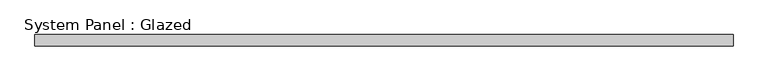
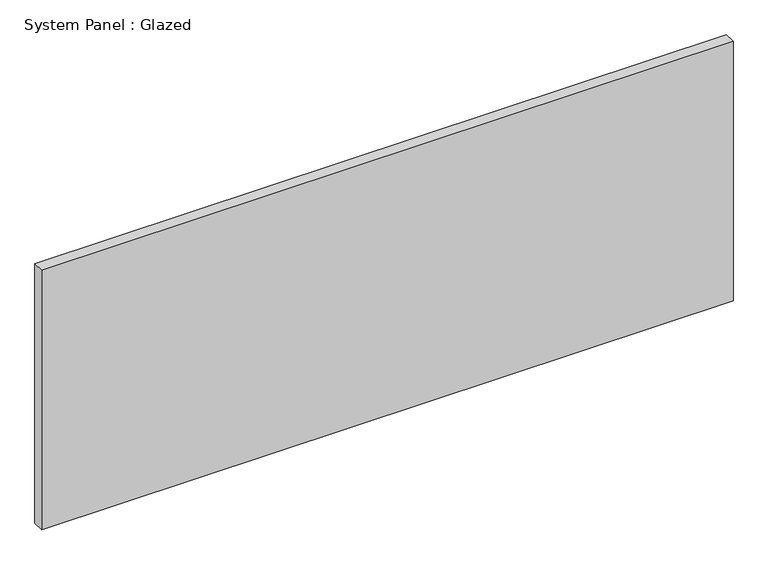
"""IFC4 building model written with IfcOpenShell, lengths in millimetres: plate geometry, System Panel : Glazed."""

import ifcopenshell
import ifcopenshell.guid

model = None  # the IFC model being written
_history = None  # IfcOwnerHistory: only IFC2X3 demands one
_inside = {}  # id of a spatial element -> (the spatial element, [elements in it])
_under = {}  # id of a project, library or spatial element -> (it, [spatial elements below it])
_declared = {}  # id of a project -> (the project, [libraries it declares])
_typed = {}  # id of a type object -> (the type object, [elements of that type])
_made_of = {}  # id of a material, layer set ... -> (it, [elements and type objects made of it])


def new_model(schema):
    """Start an empty IFC model of exactly this schema.

    Asked for "IFC4X3", IfcOpenShell would pick the latest addendum, in which some entities
    have other attributes; the version numbers below select the first issue.
    IFC2X3 requires an IfcOwnerHistory on every rooted entity: one is made here for all.
    """
    global model, _history
    if schema == "IFC4X3":
        model = ifcopenshell.file(schema_version=(4, 3, 0, 0))
    else:
        model = ifcopenshell.file(schema=schema)
    _inside.clear()
    _under.clear()
    _declared.clear()
    _typed.clear()
    _made_of.clear()
    _history = None
    if model.schema == "IFC2X3":
        org = make("IfcOrganization", Name="unknown")
        user = make(
            "IfcPersonAndOrganization",
            ThePerson=make("IfcPerson", FamilyName="unknown"),
            TheOrganization=org,
        )
        app = make(
            "IfcApplication",
            ApplicationDeveloper=org,
            Version="unknown",
            ApplicationFullName="unknown",
            ApplicationIdentifier="unknown",
        )
        _history = make(
            "IfcOwnerHistory",
            OwningUser=user,
            OwningApplication=app,
            ChangeAction="ADDED",
            CreationDate=0,
        )
    return model


def make(cls, **values):
    """One entity of the class cls with the attributes given. An attribute that is None is left unset."""
    return model.create_entity(
        cls, **{name: value for name, value in values.items() if value is not None}
    )


def rooted(cls, **values):
    """An entity with a GlobalId (a new one), such as an element, a storey or a relation."""
    return make(cls, GlobalId=ifcopenshell.guid.new(), OwnerHistory=_history, **values)


def si_unit(unit_type, name, prefix=None):
    """IfcSIUnit, for example si_unit("LENGTHUNIT", "METRE", prefix="MILLI")."""
    return make("IfcSIUnit", UnitType=unit_type, Prefix=prefix, Name=name)


def assignment(units):
    """IfcUnitAssignment: the units of a project."""
    return None if units is None else make("IfcUnitAssignment", Units=units)


def point(xyz):
    """IfcCartesianPoint."""
    return None if xyz is None else make("IfcCartesianPoint", Coordinates=xyz)


def direction(xyz):
    """IfcDirection."""
    return None if xyz is None else make("IfcDirection", DirectionRatios=xyz)


def frame(location, z_axis=None, x_axis=None):
    """IfcAxis2Placement3D, a coordinate frame: its origin and axes. An axis left out is left unset."""
    return make(
        "IfcAxis2Placement3D",
        Location=point(location),
        Axis=direction(z_axis),
        RefDirection=direction(x_axis),
    )


def origin():
    """The frame at (0, 0, 0) with its axes left unset."""
    return frame((0.0, 0.0, 0.0))


def origin_with_axes():
    """The frame at (0, 0, 0) with the z axis (0, 0, 1) and the x axis (1, 0, 0) written out."""
    return frame((0.0, 0.0, 0.0), z_axis=(0.0, 0.0, 1.0), x_axis=(1.0, 0.0, 0.0))


def place(relative_to, where):
    """IfcLocalPlacement: puts the frame where relative to a parent placement (None: the world)."""
    return make(
        "IfcLocalPlacement", PlacementRelTo=relative_to, RelativePlacement=where
    )


def context(
    kind, dimensions, precision=None, world=None, true_north=None, identifier=None
):
    """IfcGeometricRepresentationContext, for example the 3D "Model" context."""
    return make(
        "IfcGeometricRepresentationContext",
        ContextIdentifier=identifier,
        ContextType=kind,
        CoordinateSpaceDimension=dimensions,
        Precision=precision,
        WorldCoordinateSystem=world,
        TrueNorth=true_north,
    )


def project(units=None, contexts=None):
    """IfcProject with its units and contexts."""
    return rooted(
        "IfcProject",
        Name="project",
        RepresentationContexts=contexts,
        UnitsInContext=assignment(units),
    )


def spatial(cls, under=None, at=None, **own):
    """A site, building, storey or space (cls), placed at a placement, below another one or the project."""
    s = rooted(cls, ObjectPlacement=at, **own)
    if under is not None:
        _under.setdefault(under.id(), (under, []))[1].append(s)
    return s


def polyline(points):
    """IfcPolyline through the points."""
    return make("IfcPolyline", Points=[point(p) for p in points])


def outline(outer, holes=None, kind="AREA"):
    """IfcArbitraryClosedProfileDef: a profile drawn as a closed curve; with holes, ...WithVoids."""
    if holes is None:
        return make("IfcArbitraryClosedProfileDef", ProfileType=kind, OuterCurve=outer)
    return make(
        "IfcArbitraryProfileDefWithVoids",
        ProfileType=kind,
        OuterCurve=outer,
        InnerCurves=holes,
    )


def extrude(swept, where, along, depth):
    """IfcExtrudedAreaSolid: the profile swept, set in the frame where, extruded along a direction by depth."""
    return make(
        "IfcExtrudedAreaSolid",
        SweptArea=swept,
        Position=where,
        ExtrudedDirection=direction(along),
        Depth=depth,
    )


def shape(context_of_items, identifier, shape_type, items):
    """IfcShapeRepresentation: the items that make up one representation, for example the "Body"."""
    return make(
        "IfcShapeRepresentation",
        ContextOfItems=context_of_items,
        RepresentationIdentifier=identifier,
        RepresentationType=shape_type,
        Items=items,
    )


def source(mapping_origin, context_of_items, identifier, shape_type, items):
    """IfcRepresentationMap: a shape defined once, which mapped items show again and again."""
    return make(
        "IfcRepresentationMap",
        MappingOrigin=mapping_origin,
        MappedRepresentation=shape(context_of_items, identifier, shape_type, items),
    )


def transform(
    local_origin,
    x_axis=None,
    y_axis=None,
    z_axis=None,
    scale=None,
    scale2=None,
    scale3=None,
    uniform=True,
):
    """IfcCartesianTransformationOperator3D, or its non-uniform kind. x_axis, y_axis, z_axis: its Axis1, 2, 3."""
    if uniform:
        return make(
            "IfcCartesianTransformationOperator3D",
            Axis1=direction(x_axis),
            Axis2=direction(y_axis),
            LocalOrigin=point(local_origin),
            Scale=scale,
            Axis3=direction(z_axis),
        )
    return make(
        "IfcCartesianTransformationOperator3DnonUniform",
        Axis1=direction(x_axis),
        Axis2=direction(y_axis),
        LocalOrigin=point(local_origin),
        Scale=scale,
        Axis3=direction(z_axis),
        Scale2=scale2,
        Scale3=scale3,
    )


def mapped(mapping_source, mapping_target):
    """IfcMappedItem: shows the shape of a source again, moved by a transform."""
    return make(
        "IfcMappedItem", MappingSource=mapping_source, MappingTarget=mapping_target
    )


def made_of(thing, what):
    """Note that an element or type object is made of a material, layer set ...; save() writes the relation."""
    if what is not None:
        _made_of.setdefault(what.id(), (what, []))[1].append(thing)
    return thing


def element(
    cls,
    number,
    at=None,
    inside=None,
    cuts=None,
    type_object=None,
    material=None,
    context=None,
    identifier="Body",
    shape_type=None,
    held_by="IfcProductDefinitionShape",
    body=None,
    shapes=None,
    **own,
):
    """One element of the class cls, such as IfcWall. Its Tag is "e" and its number.

    at: its placement. inside: the storey or other place that contains it. cuts: it is an
    opening in that element (IfcRelVoidsElement). A single representation is given by context,
    identifier, shape_type and body (its items); several are given by shapes. held_by: the class
    of the entity that holds the representations. save() writes the other relations.
    """
    e = rooted(cls, Tag="e%d" % number, ObjectPlacement=at, **own)
    if body is not None:
        shapes = [shape(context, identifier, shape_type, body)]
    if shapes is not None:
        e.Representation = make(held_by, Representations=shapes)
    if inside is not None:
        _inside.setdefault(inside.id(), (inside, []))[1].append(e)
    if cuts is not None:
        rooted(
            "IfcRelVoidsElement", RelatingBuildingElement=cuts, RelatedOpeningElement=e
        )
    if type_object is not None:
        _typed.setdefault(type_object.id(), (type_object, []))[1].append(e)
    return made_of(e, material)


def aggregate(whole, parts):
    """IfcRelAggregates: a whole, such as a stair, and the parts it consists of."""
    return rooted("IfcRelAggregates", RelatingObject=whole, RelatedObjects=parts)


def save(model, path):
    """Write the relations noted so far, then the file.

    IfcRelAggregates (storeys below a building ...), IfcRelContainedInSpatialStructure (elements
    in a storey), IfcRelDefinesByType, IfcRelAssociatesMaterial and IfcRelDeclares: one each for
    every whole, place, type object, material and project.
    """
    for whole, parts in _under.values():
        aggregate(whole, parts)
    for where, things in _inside.values():
        rooted(
            "IfcRelContainedInSpatialStructure",
            RelatedElements=things,
            RelatingStructure=where,
        )
    for kind, things in _typed.values():
        rooted("IfcRelDefinesByType", RelatedObjects=things, RelatingType=kind)
    for what, things in _made_of.values():
        rooted("IfcRelAssociatesMaterial", RelatedObjects=things, RelatingMaterial=what)
    for by, libraries in _declared.values():
        rooted("IfcRelDeclares", RelatingContext=by, RelatedDefinitions=libraries)
    model.write(path)


def system_panel_glazed_956e323c(model_context):
    return source(origin(), model_context, "Body", "SweptSolid", [
        extrude(outline(polyline([(768.35, 19.05), (-768.35, 19.05), (-768.35, 44.45), (768.35, 44.45), (768.35, 19.05)])), origin_with_axes(), (0.0, 0.0, 1.0), 609.6),
    ])


if __name__ == "__main__":
    model = new_model("IFC4")
    model_context = context("Model", 3, world=origin())
    ifc_project = project(units=[si_unit("LENGTHUNIT", "METRE", prefix="MILLI")], contexts=[model_context])
    site = spatial("IfcSite", under=ifc_project)
    building = spatial("IfcBuilding", under=site)
    placement = place(None, origin())
    system_panel_glazed_shape = system_panel_glazed_956e323c(model_context)
    element("IfcPlate", 1, ObjectType="System Panel : Glazed", at=placement, inside=building, context=model_context, shape_type="MappedRepresentation", body=[
        mapped(system_panel_glazed_shape, transform((0.0, 0.0, 0.0), x_axis=(1.0, 0.0, 0.0), y_axis=(0.0, 1.0, 0.0), z_axis=(0.0, 0.0, 1.0))),
    ])
    save(model, "model.ifc")

# Revit data of these elements
# Element 1 (IfcPlate, "System Panel : Glazed")
#   Materials on its faces: "Glass"
# Materials
#   "Glass": class "Glass", colour RGB 0 128 192, transparency 0.75
